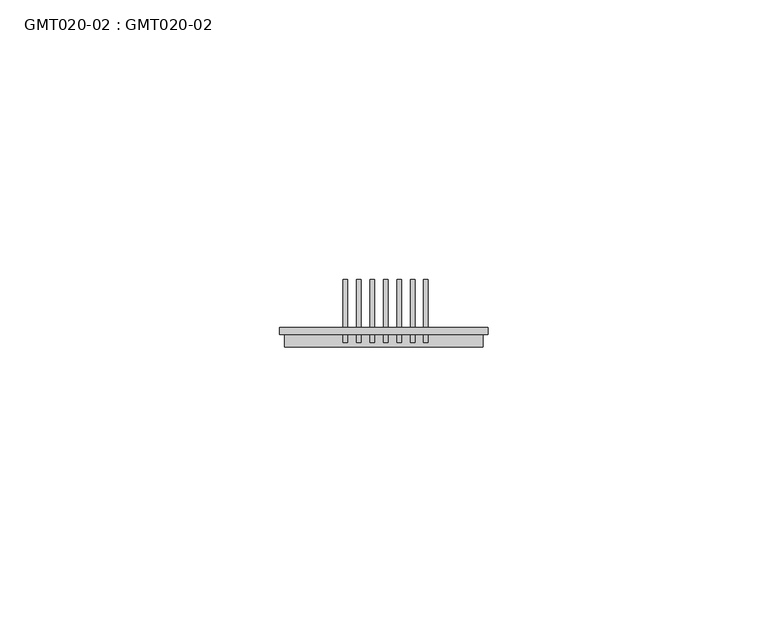
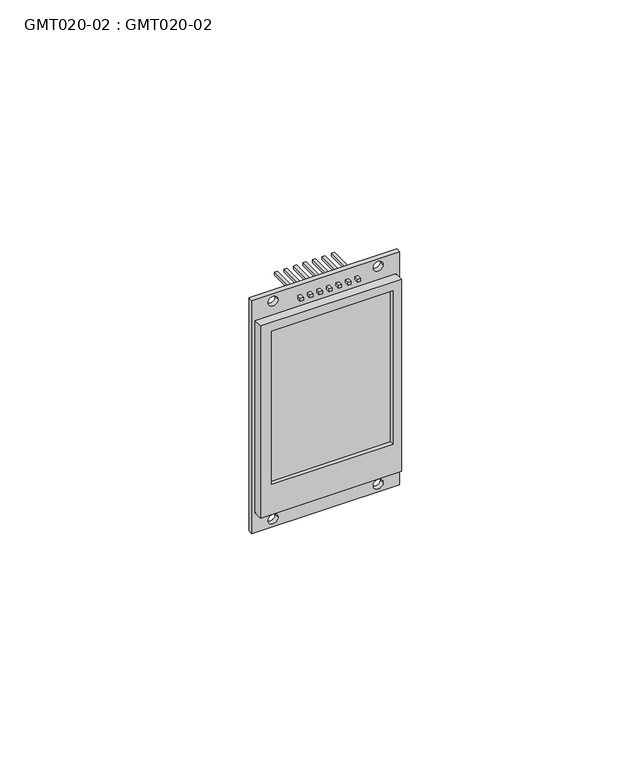
"""IFC4 building model written with IfcOpenShell, lengths in millimetres: furniture geometry, GMT020-02 : GMT020-02."""

import ifcopenshell
import ifcopenshell.guid

model = None  # the IFC model being written
_history = None  # IfcOwnerHistory: only IFC2X3 demands one
_inside = {}  # id of a spatial element -> (the spatial element, [elements in it])
_under = {}  # id of a project, library or spatial element -> (it, [spatial elements below it])
_declared = {}  # id of a project -> (the project, [libraries it declares])
_typed = {}  # id of a type object -> (the type object, [elements of that type])
_made_of = {}  # id of a material, layer set ... -> (it, [elements and type objects made of it])


def new_model(schema):
    """Start an empty IFC model of exactly this schema.

    Asked for "IFC4X3", IfcOpenShell would pick the latest addendum, in which some entities
    have other attributes; the version numbers below select the first issue.
    IFC2X3 requires an IfcOwnerHistory on every rooted entity: one is made here for all.
    """
    global model, _history
    if schema == "IFC4X3":
        model = ifcopenshell.file(schema_version=(4, 3, 0, 0))
    else:
        model = ifcopenshell.file(schema=schema)
    _inside.clear()
    _under.clear()
    _declared.clear()
    _typed.clear()
    _made_of.clear()
    _history = None
    if model.schema == "IFC2X3":
        org = make("IfcOrganization", Name="unknown")
        user = make(
            "IfcPersonAndOrganization",
            ThePerson=make("IfcPerson", FamilyName="unknown"),
            TheOrganization=org,
        )
        app = make(
            "IfcApplication",
            ApplicationDeveloper=org,
            Version="unknown",
            ApplicationFullName="unknown",
            ApplicationIdentifier="unknown",
        )
        _history = make(
            "IfcOwnerHistory",
            OwningUser=user,
            OwningApplication=app,
            ChangeAction="ADDED",
            CreationDate=0,
        )
    return model


def make(cls, **values):
    """One entity of the class cls with the attributes given. An attribute that is None is left unset."""
    return model.create_entity(
        cls, **{name: value for name, value in values.items() if value is not None}
    )


def rooted(cls, **values):
    """An entity with a GlobalId (a new one), such as an element, a storey or a relation."""
    return make(cls, GlobalId=ifcopenshell.guid.new(), OwnerHistory=_history, **values)


def si_unit(unit_type, name, prefix=None):
    """IfcSIUnit, for example si_unit("LENGTHUNIT", "METRE", prefix="MILLI")."""
    return make("IfcSIUnit", UnitType=unit_type, Prefix=prefix, Name=name)


def assignment(units):
    """IfcUnitAssignment: the units of a project."""
    return None if units is None else make("IfcUnitAssignment", Units=units)


def point(xyz):
    """IfcCartesianPoint."""
    return None if xyz is None else make("IfcCartesianPoint", Coordinates=xyz)


def direction(xyz):
    """IfcDirection."""
    return None if xyz is None else make("IfcDirection", DirectionRatios=xyz)


def frame(location, z_axis=None, x_axis=None):
    """IfcAxis2Placement3D, a coordinate frame: its origin and axes. An axis left out is left unset."""
    return make(
        "IfcAxis2Placement3D",
        Location=point(location),
        Axis=direction(z_axis),
        RefDirection=direction(x_axis),
    )


def origin():
    """The frame at (0, 0, 0) with its axes left unset."""
    return frame((0.0, 0.0, 0.0))


def place(relative_to, where):
    """IfcLocalPlacement: puts the frame where relative to a parent placement (None: the world)."""
    return make(
        "IfcLocalPlacement", PlacementRelTo=relative_to, RelativePlacement=where
    )


def context(
    kind, dimensions, precision=None, world=None, true_north=None, identifier=None
):
    """IfcGeometricRepresentationContext, for example the 3D "Model" context."""
    return make(
        "IfcGeometricRepresentationContext",
        ContextIdentifier=identifier,
        ContextType=kind,
        CoordinateSpaceDimension=dimensions,
        Precision=precision,
        WorldCoordinateSystem=world,
        TrueNorth=true_north,
    )


def project(units=None, contexts=None):
    """IfcProject with its units and contexts."""
    return rooted(
        "IfcProject",
        Name="project",
        RepresentationContexts=contexts,
        UnitsInContext=assignment(units),
    )


def spatial(cls, under=None, at=None, **own):
    """A site, building, storey or space (cls), placed at a placement, below another one or the project."""
    s = rooted(cls, ObjectPlacement=at, **own)
    if under is not None:
        _under.setdefault(under.id(), (under, []))[1].append(s)
    return s


def polyline(points):
    """IfcPolyline through the points."""
    return make("IfcPolyline", Points=[point(p) for p in points])


def circle_curve(where, radius):
    """IfcCircle in the frame where."""
    return make("IfcCircle", Position=where, Radius=radius)


def outline(outer, holes=None, kind="AREA"):
    """IfcArbitraryClosedProfileDef: a profile drawn as a closed curve; with holes, ...WithVoids."""
    if holes is None:
        return make("IfcArbitraryClosedProfileDef", ProfileType=kind, OuterCurve=outer)
    return make(
        "IfcArbitraryProfileDefWithVoids",
        ProfileType=kind,
        OuterCurve=outer,
        InnerCurves=holes,
    )


def extrude(swept, where, along, depth):
    """IfcExtrudedAreaSolid: the profile swept, set in the frame where, extruded along a direction by depth."""
    return make(
        "IfcExtrudedAreaSolid",
        SweptArea=swept,
        Position=where,
        ExtrudedDirection=direction(along),
        Depth=depth,
    )


def shape(context_of_items, identifier, shape_type, items):
    """IfcShapeRepresentation: the items that make up one representation, for example the "Body"."""
    return make(
        "IfcShapeRepresentation",
        ContextOfItems=context_of_items,
        RepresentationIdentifier=identifier,
        RepresentationType=shape_type,
        Items=items,
    )


def source(mapping_origin, context_of_items, identifier, shape_type, items):
    """IfcRepresentationMap: a shape defined once, which mapped items show again and again."""
    return make(
        "IfcRepresentationMap",
        MappingOrigin=mapping_origin,
        MappedRepresentation=shape(context_of_items, identifier, shape_type, items),
    )


def transform(
    local_origin,
    x_axis=None,
    y_axis=None,
    z_axis=None,
    scale=None,
    scale2=None,
    scale3=None,
    uniform=True,
):
    """IfcCartesianTransformationOperator3D, or its non-uniform kind. x_axis, y_axis, z_axis: its Axis1, 2, 3."""
    if uniform:
        return make(
            "IfcCartesianTransformationOperator3D",
            Axis1=direction(x_axis),
            Axis2=direction(y_axis),
            LocalOrigin=point(local_origin),
            Scale=scale,
            Axis3=direction(z_axis),
        )
    return make(
        "IfcCartesianTransformationOperator3DnonUniform",
        Axis1=direction(x_axis),
        Axis2=direction(y_axis),
        LocalOrigin=point(local_origin),
        Scale=scale,
        Axis3=direction(z_axis),
        Scale2=scale2,
        Scale3=scale3,
    )


def mapped(mapping_source, mapping_target):
    """IfcMappedItem: shows the shape of a source again, moved by a transform."""
    return make(
        "IfcMappedItem", MappingSource=mapping_source, MappingTarget=mapping_target
    )


def made_of(thing, what):
    """Note that an element or type object is made of a material, layer set ...; save() writes the relation."""
    if what is not None:
        _made_of.setdefault(what.id(), (what, []))[1].append(thing)
    return thing


def element(
    cls,
    number,
    at=None,
    inside=None,
    cuts=None,
    type_object=None,
    material=None,
    context=None,
    identifier="Body",
    shape_type=None,
    held_by="IfcProductDefinitionShape",
    body=None,
    shapes=None,
    **own,
):
    """One element of the class cls, such as IfcWall. Its Tag is "e" and its number.

    at: its placement. inside: the storey or other place that contains it. cuts: it is an
    opening in that element (IfcRelVoidsElement). A single representation is given by context,
    identifier, shape_type and body (its items); several are given by shapes. held_by: the class
    of the entity that holds the representations. save() writes the other relations.
    """
    e = rooted(cls, Tag="e%d" % number, ObjectPlacement=at, **own)
    if body is not None:
        shapes = [shape(context, identifier, shape_type, body)]
    if shapes is not None:
        e.Representation = make(held_by, Representations=shapes)
    if inside is not None:
        _inside.setdefault(inside.id(), (inside, []))[1].append(e)
    if cuts is not None:
        rooted(
            "IfcRelVoidsElement", RelatingBuildingElement=cuts, RelatedOpeningElement=e
        )
    if type_object is not None:
        _typed.setdefault(type_object.id(), (type_object, []))[1].append(e)
    return made_of(e, material)


def aggregate(whole, parts):
    """IfcRelAggregates: a whole, such as a stair, and the parts it consists of."""
    return rooted("IfcRelAggregates", RelatingObject=whole, RelatedObjects=parts)


def save(model, path):
    """Write the relations noted so far, then the file.

    IfcRelAggregates (storeys below a building ...), IfcRelContainedInSpatialStructure (elements
    in a storey), IfcRelDefinesByType, IfcRelAssociatesMaterial and IfcRelDeclares: one each for
    every whole, place, type object, material and project.
    """
    for whole, parts in _under.values():
        aggregate(whole, parts)
    for where, things in _inside.values():
        rooted(
            "IfcRelContainedInSpatialStructure",
            RelatedElements=things,
            RelatingStructure=where,
        )
    for kind, things in _typed.values():
        rooted("IfcRelDefinesByType", RelatedObjects=things, RelatingType=kind)
    for what, things in _made_of.values():
        rooted("IfcRelAssociatesMaterial", RelatedObjects=things, RelatingMaterial=what)
    for by, libraries in _declared.values():
        rooted("IfcRelDeclares", RelatingContext=by, RelatedDefinitions=libraries)
    model.write(path)


def plane_surface(at):
    """IfcPlane: the flat surface through the origin of the frame at, square to its z axis."""
    return make("IfcPlane", Position=at)


def revolved_surface(curve, axis_point, axis_direction):
    """IfcSurfaceOfRevolution: the curve turned about the line through axis_point along axis_direction."""
    return make(
        "IfcSurfaceOfRevolution",
        SweptCurve=make("IfcArbitraryOpenProfileDef", ProfileType="CURVE", Curve=curve),
        AxisPosition=make("IfcAxis1Placement", Location=point(axis_point), Axis=direction(axis_direction)),
    )


def advanced_brep(points, edges, surfaces, faces):
    """IfcAdvancedBrep: a solid bounded by faces that lie on surfaces and meet in shared edges.

    An edge is (start, end): straight between two places in points (the first is 0);
    or (start, end, curve); or (start, end, curve, False) where it runs against its curve.
    A face is (place in surfaces, loops), or (place, loops, False) where it looks against
    its surface's normal. A loop lists edges by number (the first is 1), with a minus sign
    where the edge is run from its end to its start. The first loop is the outer one.
    """
    corners = [point(p) for p in points]
    vertices = [make("IfcVertexPoint", VertexGeometry=c) for c in corners]
    made = []
    for start, end, *more in edges:
        made.append(
            make(
                "IfcEdgeCurve",
                EdgeStart=vertices[start],
                EdgeEnd=vertices[end],
                EdgeGeometry=more[0] if more else make("IfcPolyline", Points=[corners[start], corners[end]]),
                SameSense=more[1] if len(more) > 1 else True,
            )
        )
    hull = []
    for where, loops, *sense in faces:
        bounds = []
        for j, loop in enumerate(loops):
            ring = [make("IfcOrientedEdge", EdgeElement=made[abs(k) - 1], Orientation=k > 0) for k in loop]
            bounds.append(
                make(
                    "IfcFaceOuterBound" if j == 0 else "IfcFaceBound",
                    Bound=make("IfcEdgeLoop", EdgeList=ring),
                    Orientation=True,
                )
            )
        hull.append(make("IfcAdvancedFace", Bounds=bounds, FaceSurface=surfaces[where], SameSense=sense[0] if sense else True))
    return make("IfcAdvancedBrep", Outer=make("IfcClosedShell", CfsFaces=hull))


def gmt020_02_gmt020_02_ca843257(model_context):
    return source(origin(), model_context, "Body", "SolidModel", [
        advanced_brep(
        [(18.3, -32.2, 62.0), (18.3, -31.0, 62.0), (-19.0, -31.0, 62.0), (-19.0, -32.2, 62.0), (18.3, -32.2, 0.0), (-19.0, -32.2, 0.0), (-19.0, -31.0, 0.0), (18.3, -31.0, 0.0), (-14.85, -31.0, 60.0), (-12.35, -31.0, 60.0), (-14.85, -31.0, 2.0), (-12.35, -31.0, 2.0), (14.15, -31.0, 60.0), (11.65, -31.0, 60.0), (14.15, -31.0, 2.0), (11.65, -31.0, 2.0), (-18.1, -32.2, 56.4), (17.4, -32.2, 56.4), (17.4, -32.2, 5.2), (-18.1, -32.2, 5.2), (-12.35, -32.2, 60.0), (-14.85, -32.2, 60.0), (-12.35, -32.2, 2.0), (-14.85, -32.2, 2.0), (11.65, -32.2, 60.0), (14.15, -32.2, 60.0), (11.65, -32.2, 2.0), (14.15, -32.2, 2.0), (17.4, -34.4693991, 56.4), (-18.1, -34.4693991, 56.4), (17.4, -34.4693991, 5.2), (-18.1, -34.4693991, 5.2), (-15.3, -34.4693991, 54.0), (15.3, -34.4693991, 54.0), (15.3, -34.4693991, 13.2), (-15.3, -34.4693991, 13.2), (-15.3, -33.4693991, 54.0), (15.3, -33.4693991, 54.0), (15.3, -33.4693991, 13.2), (-15.3, -33.4693991, 13.2)],
        [
            (0, 1),
            (1, 2),
            (2, 3),
            (3, 0),
            (4, 5),
            (5, 6),
            (6, 7),
            (7, 4),
            (0, 4),
            (7, 1),
            (6, 2),
            (8, 9, circle_curve(frame((-13.6, -31.0, 60.0), z_axis=(0.0, -1.0, 0.0), x_axis=(1.0, 0.0, 0.0)), 1.25)),
            (9, 8, circle_curve(frame((-13.6, -31.0, 60.0), z_axis=(0.0, -1.0, 0.0), x_axis=(1.0, 0.0, 0.0)), 1.25)),
            (10, 11, circle_curve(frame((-13.6, -31.0, 2.0), z_axis=(0.0, -1.0, 0.0), x_axis=(1.0, 0.0, 0.0)), 1.25)),
            (11, 10, circle_curve(frame((-13.6, -31.0, 2.0), z_axis=(0.0, -1.0, 0.0), x_axis=(1.0, 0.0, 0.0)), 1.25)),
            (12, 13, circle_curve(frame((12.9, -31.0, 60.0), z_axis=(0.0, -1.0, 0.0), x_axis=(-1.0, 0.0, 0.0)), 1.25)),
            (13, 12, circle_curve(frame((12.9, -31.0, 60.0), z_axis=(0.0, -1.0, 0.0), x_axis=(-1.0, 0.0, 0.0)), 1.25)),
            (14, 15, circle_curve(frame((12.9, -31.0, 2.0), z_axis=(0.0, -1.0, 0.0), x_axis=(-1.0, 0.0, 0.0)), 1.25)),
            (15, 14, circle_curve(frame((12.9, -31.0, 2.0), z_axis=(0.0, -1.0, 0.0), x_axis=(-1.0, 0.0, 0.0)), 1.25)),
            (5, 3),
            (16, 17),
            (17, 18),
            (18, 19),
            (19, 16),
            (20, 21, circle_curve(frame((-13.6, -32.2, 60.0), z_axis=(0.0, 1.0, 0.0), x_axis=(1.0, 0.0, 0.0)), 1.25)),
            (21, 20, circle_curve(frame((-13.6, -32.2, 60.0), z_axis=(0.0, 1.0, 0.0), x_axis=(1.0, 0.0, 0.0)), 1.25)),
            (22, 23, circle_curve(frame((-13.6, -32.2, 2.0), z_axis=(0.0, 1.0, 0.0), x_axis=(1.0, 0.0, 0.0)), 1.25)),
            (23, 22, circle_curve(frame((-13.6, -32.2, 2.0), z_axis=(0.0, 1.0, 0.0), x_axis=(1.0, 0.0, 0.0)), 1.25)),
            (24, 25, circle_curve(frame((12.9, -32.2, 60.0), z_axis=(0.0, 1.0, 0.0), x_axis=(-1.0, 0.0, 0.0)), 1.25)),
            (25, 24, circle_curve(frame((12.9, -32.2, 60.0), z_axis=(0.0, 1.0, 0.0), x_axis=(-1.0, 0.0, 0.0)), 1.25)),
            (26, 27, circle_curve(frame((12.9, -32.2, 2.0), z_axis=(0.0, 1.0, 0.0), x_axis=(-1.0, 0.0, 0.0)), 1.25)),
            (27, 26, circle_curve(frame((12.9, -32.2, 2.0), z_axis=(0.0, 1.0, 0.0), x_axis=(-1.0, 0.0, 0.0)), 1.25)),
            (28, 17),
            (16, 29),
            (29, 28),
            (30, 31),
            (31, 19),
            (18, 30),
            (28, 30),
            (31, 29),
            (32, 33),
            (33, 34),
            (34, 35),
            (35, 32),
            (8, 21),
            (20, 9),
            (10, 23),
            (22, 11),
            (32, 36),
            (36, 37),
            (37, 33),
            (34, 38),
            (38, 39),
            (39, 35),
            (37, 38),
            (36, 39),
            (12, 25),
            (24, 13),
            (14, 27),
            (26, 15),
        ],
        [
            plane_surface(frame((18.3, -32.2, 62.0), z_axis=(0.0, 0.0, 1.0), x_axis=(0.0, 1.0, 0.0))),
            plane_surface(frame((18.3, -32.2, 0.0), z_axis=(0.0, 0.0, -1.0), x_axis=(0.0, -1.0, 0.0))),
            plane_surface(frame((18.3, -32.2, 62.0), z_axis=(1.0, 0.0, 0.0), x_axis=(0.0, 0.0, -1.0))),
            plane_surface(frame((18.3, -31.0, 62.0), z_axis=(0.0, 1.0, 0.0), x_axis=(0.0, 0.0, -1.0))),
            plane_surface(frame((-19.0, -31.0, 62.0), z_axis=(-1.0, 0.0, 0.0), x_axis=(0.0, 0.0, -1.0))),
            plane_surface(frame((-19.0, -32.2, 62.0), z_axis=(0.0, -1.0, 0.0), x_axis=(0.0, 0.0, -1.0))),
            plane_surface(frame((17.4, -33.4693991, 56.4), z_axis=(0.0, 0.0, 1.0), x_axis=(0.0, 1.0, 0.0))),
            plane_surface(frame((17.4, -33.4693991, 5.2), z_axis=(0.0, 0.0, -1.0), x_axis=(0.0, -1.0, 0.0))),
            plane_surface(frame((17.4, -34.4693991, 56.4), z_axis=(1.0, 0.0, 0.0), x_axis=(0.0, 0.0, -1.0))),
            plane_surface(frame((-18.1, -32.2693991, 56.4), z_axis=(-1.0, 0.0, 0.0), x_axis=(0.0, 0.0, -1.0))),
            plane_surface(frame((-18.1, -34.4693991, 56.4), z_axis=(0.0, -1.0, 0.0), x_axis=(0.0, 0.0, -1.0))),
            revolved_surface(polyline([(-12.35, -32.2, 60.0), (-12.35, -31.0, 60.0)]), (-13.6, -28.9796632, 60.0), (0.0, -1.0, 0.0)),
            revolved_surface(polyline([(-12.35, -32.2, 2.0), (-12.35, -31.0, 2.0)]), (-13.6, -28.9796632, 2.0), (0.0, -1.0, 0.0)),
            plane_surface(frame((15.3, -34.4, 54.0), z_axis=(0.0, 0.0, -1.0), x_axis=(0.0, 1.0, 0.0))),
            plane_surface(frame((15.3, -34.4, 13.2), z_axis=(0.0, 0.0, 1.0), x_axis=(0.0, -1.0, 0.0))),
            plane_surface(frame((15.3, -34.4693991, 54.0), z_axis=(-1.0, 0.0, 0.0), x_axis=(0.0, 0.0, -1.0))),
            plane_surface(frame((15.3, -33.4693991, 54.0), z_axis=(0.0, -1.0, 0.0), x_axis=(0.0, 0.0, -1.0))),
            plane_surface(frame((-15.3, -33.4693991, 54.0), z_axis=(1.0, 0.0, 0.0), x_axis=(0.0, 0.0, -1.0))),
            revolved_surface(polyline([(11.65, -32.2, 60.0), (11.65, -31.0, 60.0)]), (12.9, -31.0, 60.0), (0.0, -1.0, 0.0)),
            revolved_surface(polyline([(11.65, -32.2, 2.0), (11.65, -31.0, 2.0)]), (12.9, -31.0, 2.0), (0.0, -1.0, 0.0)),
        ],
        [
            (0, [[1, 2, 3, 4]]),
            (1, [[5, 6, 7, 8]]),
            (2, [[-1, 9, -8, 10]]),
            (3, [[-2, -10, -7, 11], [12, 13], [14, 15], [16, 17], [18, 19]]),
            (4, [[-3, -11, -6, 20]]),
            (5, [[-4, -20, -5, -9], [21, 22, 23, 24], [25, 26], [27, 28], [29, 30], [31, 32]]),
            (6, [[33, -21, 34, 35]]),
            (7, [[36, 37, -23, 38]]),
            (8, [[-33, 39, -38, -22]]),
            (9, [[-34, -24, -37, 40]]),
            (10, [[-35, -40, -36, -39], [41, 42, 43, 44]]),
            (11, [[45, -25, 46, -12]]),
            (11, [[-45, -13, -46, -26]]),
            (12, [[47, -27, 48, -14]]),
            (12, [[-47, -15, -48, -28]]),
            (13, [[49, 50, 51, -41]]),
            (14, [[52, 53, 54, -43]]),
            (15, [[-51, 55, -52, -42]]),
            (16, [[-50, 56, -53, -55]]),
            (17, [[-49, -44, -54, -56]]),
            (18, [[57, -29, 58, -16]]),
            (18, [[-57, -17, -58, -30]]),
            (19, [[59, -31, 60, -18]]),
            (19, [[-59, -19, -60, -32]]),
        ],
    ),
        extrude(outline(polyline([(-7.6, -33.6693991), (-7.6, -22.3693991), (-6.8, -22.3693991), (-6.8, -33.6693991), (-7.6, -33.6693991)])), frame((0.0, 0.0, 58.8), z_axis=(0.0, 0.0, 1.0), x_axis=(1.0, 0.0, 0.0)), (0.0, 0.0, 1.0), 0.8),
        extrude(outline(polyline([(6.8, -33.6693991), (6.8, -22.3693991), (7.6, -22.3693991), (7.6, -33.6693991), (6.8, -33.6693991)])), frame((0.0, 0.0, 58.8), z_axis=(0.0, 0.0, 1.0), x_axis=(1.0, 0.0, 0.0)), (0.0, 0.0, 1.0), 0.8),
        extrude(outline(polyline([(4.4, -33.6693991), (4.4, -22.3693991), (5.2, -22.3693991), (5.2, -33.6693991), (4.4, -33.6693991)])), frame((0.0, 0.0, 58.8), z_axis=(0.0, 0.0, 1.0), x_axis=(1.0, 0.0, 0.0)), (0.0, 0.0, 1.0), 0.8),
        extrude(outline(polyline([(2.0, -33.6693991), (2.0, -22.3693991), (2.8, -22.3693991), (2.8, -33.6693991), (2.0, -33.6693991)])), frame((0.0, 0.0, 58.8), z_axis=(0.0, 0.0, 1.0), x_axis=(1.0, 0.0, 0.0)), (0.0, 0.0, 1.0), 0.8),
        extrude(outline(polyline([(-0.4, -33.6693991), (-0.4, -22.3693991), (0.4, -22.3693991), (0.4, -33.6693991), (-0.4, -33.6693991)])), frame((0.0, 0.0, 58.8), z_axis=(0.0, 0.0, 1.0), x_axis=(1.0, 0.0, 0.0)), (0.0, 0.0, 1.0), 0.8),
        extrude(outline(polyline([(-2.8, -33.6693991), (-2.8, -22.3693991), (-2.0, -22.3693991), (-2.0, -33.6693991), (-2.8, -33.6693991)])), frame((0.0, 0.0, 58.8), z_axis=(0.0, 0.0, 1.0), x_axis=(1.0, 0.0, 0.0)), (0.0, 0.0, 1.0), 0.8),
        extrude(outline(polyline([(-5.2, -33.6693991), (-5.2, -22.3693991), (-4.4, -22.3693991), (-4.4, -33.6693991), (-5.2, -33.6693991)])), frame((0.0, 0.0, 58.8), z_axis=(0.0, 0.0, 1.0), x_axis=(1.0, 0.0, 0.0)), (0.0, 0.0, 1.0), 0.8),
    ])


if __name__ == "__main__":
    model = new_model("IFC4")
    model_context = context("Model", 3, world=origin())
    ifc_project = project(units=[si_unit("LENGTHUNIT", "METRE", prefix="MILLI")], contexts=[model_context])
    site = spatial("IfcSite", under=ifc_project)
    building = spatial("IfcBuilding", under=site)
    placement = place(None, origin())
    gmt020_02_gmt020_02_shape = gmt020_02_gmt020_02_ca843257(model_context)
    element("IfcFurniture", 1, ObjectType="GMT020-02 : GMT020-02", at=placement, inside=building, context=model_context, shape_type="MappedRepresentation", body=[
        mapped(gmt020_02_gmt020_02_shape, transform((0.0, 0.0, 0.0), x_axis=(1.0, 0.0, 0.0), y_axis=(0.0, 1.0, 0.0), z_axis=(0.0, 0.0, 1.0))),
    ])
    save(model, "model.ifc")

# Revit data of these elements
# Type "GMT020-02 : GMT020-02"
#   Default Elevation = 0
# Element 1 (IfcFurniture, "GMT020-02 : GMT020-02")
#   Materials on its faces: ".TELA"
# Materials
#   ".TELA": class "Vidro", colour RGB 128 128 255, transparency 0.5, Cost = 0
